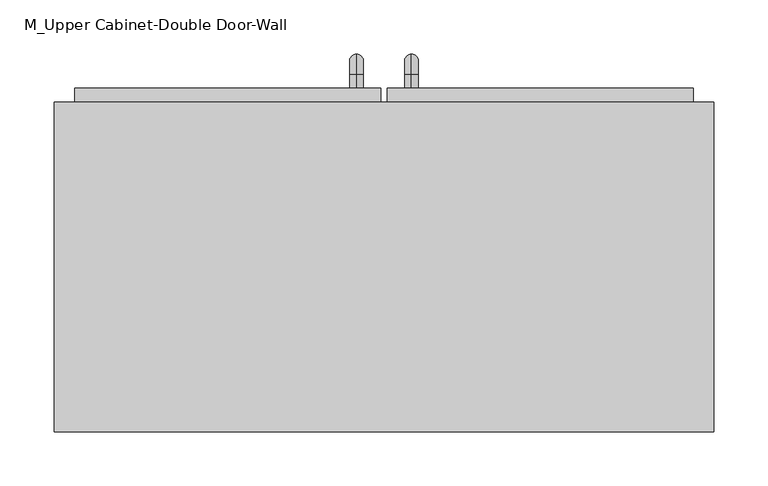
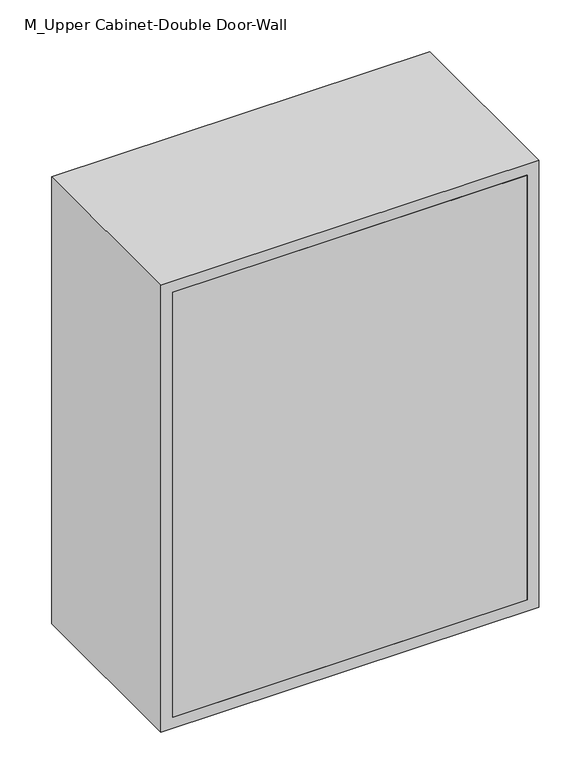
"""IFC4 building model written with IfcOpenShell, lengths in millimetres: furniture geometry, M_Upper Cabinet-Double Door-Wall : 24W X 30H."""

from ifc_helpers import new_model, si_unit, point, frame, origin, place, context, project, spatial, polyline, circle_curve, ellipse_curve, trimmed, outline, extrude, source, transform, mapped, element, save
from ifc_brep_helpers import plane_surface, cylinder_surface, revolved_surface, advanced_brep


def m_upper_cabinet_double_door_wall_c5bb5ff2(model_context):
    return source(origin(), model_context, "Body", "SolidModel", [
        advanced_brep(
        [(55.1711628, 379.4125, 1212.85), (55.1711628, 379.4125, 1225.55), (55.1711628, 392.1125, 1212.85), (55.1711628, 392.1125, 1225.55), (55.1711628, 411.1625, 1206.5), (55.1711628, 398.4625, 1206.5), (55.1711628, 398.4625, 1130.3), (55.1711628, 411.1625, 1130.3), (55.1711628, 392.1125, 1111.25), (55.1711628, 392.1125, 1123.95), (55.1711628, 379.4125, 1123.95), (55.1711628, 379.4125, 1111.25)],
        [
            (0, 1, circle_curve(frame((55.1711628, 379.4125, 1219.2), z_axis=(0.0, -1.0, 0.0), x_axis=(0.0, 0.0, -1.0)), 6.35)),
            (1, 0, circle_curve(frame((55.1711628, 379.4125, 1219.2), z_axis=(0.0, -1.0, 0.0), x_axis=(0.0, 0.0, -1.0)), 6.35)),
            (0, 2),
            (2, 3, circle_curve(frame((55.1711628, 392.1125, 1219.2), z_axis=(0.0, -1.0, 0.0), x_axis=(0.0, 0.0, -1.0)), 6.35)),
            (3, 1),
            (3, 2, circle_curve(frame((55.1711628, 392.1125, 1219.2), z_axis=(0.0, -1.0, 0.0), x_axis=(0.0, 0.0, -1.0)), 6.35)),
            (4, 3, circle_curve(frame((55.1711628, 392.1125, 1206.5), z_axis=(1.0, 0.0, 0.0), x_axis=(0.0, 0.0, 1.0)), 19.05)),
            (2, 5, circle_curve(frame((55.1711628, 392.1125, 1206.5), z_axis=(-1.0, 0.0, 0.0), x_axis=(0.0, 0.0, 1.0)), 6.35)),
            (5, 4, circle_curve(frame((55.1711628, 404.8125, 1206.5), z_axis=(0.0, 0.0, 1.0), x_axis=(0.0, -1.0, 0.0)), 6.35)),
            (4, 5, circle_curve(frame((55.1711628, 404.8125, 1206.5), z_axis=(0.0, 0.0, 1.0), x_axis=(0.0, -1.0, 0.0)), 6.35)),
            (5, 6),
            (6, 7, circle_curve(frame((55.1711628, 404.8125, 1130.3), z_axis=(0.0, 0.0, 1.0), x_axis=(0.0, -1.0, 0.0)), 6.35)),
            (7, 4),
            (7, 6, circle_curve(frame((55.1711628, 404.8125, 1130.3), z_axis=(0.0, 0.0, 1.0), x_axis=(0.0, -1.0, 0.0)), 6.35)),
            (8, 7, circle_curve(frame((55.1711628, 392.1125, 1130.3), z_axis=(1.0, 0.0, 0.0), x_axis=(0.0, 1.0, 0.0)), 19.05)),
            (6, 9, circle_curve(frame((55.1711628, 392.1125, 1130.3), z_axis=(-1.0, 0.0, 0.0), x_axis=(0.0, 1.0, 0.0)), 6.35)),
            (9, 8, circle_curve(frame((55.1711628, 392.1125, 1117.6), z_axis=(0.0, 1.0, 0.0), x_axis=(0.0, 0.0, 1.0)), 6.35)),
            (8, 9, circle_curve(frame((55.1711628, 392.1125, 1117.6), z_axis=(0.0, 1.0, 0.0), x_axis=(0.0, 0.0, 1.0)), 6.35)),
            (10, 11, circle_curve(frame((55.1711628, 379.4125, 1117.6), z_axis=(0.0, -1.0, 0.0), x_axis=(0.0, 0.0, 1.0)), 6.35)),
            (11, 10, circle_curve(frame((55.1711628, 379.4125, 1117.6), z_axis=(0.0, -1.0, 0.0), x_axis=(0.0, 0.0, 1.0)), 6.35)),
            (9, 10),
            (11, 8),
        ],
        [
            plane_surface(frame((48.8211628, 379.4125, 1219.2), z_axis=(0.0, -1.0, 0.0), x_axis=(0.0, 0.0, 1.0))),
            cylinder_surface(frame((55.1711628, 379.4125, 1219.2), z_axis=(0.0, -1.0, 0.0), x_axis=(0.0, 0.0, -1.0)), 6.35),
            revolved_surface(trimmed(ellipse_curve(frame((55.1711628, 392.1125, 1219.2), z_axis=(0.0, -1.0, 0.0), x_axis=(0.0, 0.0, -1.0)), 6.35, 6.35), [point((55.1711628, 392.1125, 1212.85))], [point((55.1711628, 392.1125, 1225.55))], True, "CARTESIAN"), (55.1711628, 392.1125, 1206.5), (-1.0, 0.0, 0.0)),
            revolved_surface(trimmed(ellipse_curve(frame((55.1711628, 392.1125, 1219.2), z_axis=(0.0, -1.0, 0.0), x_axis=(0.0, 0.0, -1.0)), 6.35, 6.35), [point((55.1711628, 392.1125, 1225.55))], [point((55.1711628, 392.1125, 1212.85))], True, "CARTESIAN"), (55.1711628, 392.1125, 1206.5), (-1.0, 0.0, 0.0)),
            cylinder_surface(frame((55.1711628, 404.8125, 1206.5), z_axis=(0.0, 0.0, 1.0), x_axis=(0.0, -1.0, 0.0)), 6.35),
            revolved_surface(trimmed(ellipse_curve(frame((55.1711628, 404.8125, 1130.3), z_axis=(0.0, 0.0, 1.0), x_axis=(0.0, -1.0, 0.0)), 6.35, 6.35), [point((55.1711628, 398.4625, 1130.3))], [point((55.1711628, 411.1625, 1130.3))], True, "CARTESIAN"), (55.1711628, 392.1125, 1130.3), (-1.0, 0.0, 0.0)),
            revolved_surface(trimmed(ellipse_curve(frame((55.1711628, 404.8125, 1130.3), z_axis=(0.0, 0.0, 1.0), x_axis=(0.0, -1.0, 0.0)), 6.35, 6.35), [point((55.1711628, 411.1625, 1130.3))], [point((55.1711628, 398.4625, 1130.3))], True, "CARTESIAN"), (55.1711628, 392.1125, 1130.3), (-1.0, 0.0, 0.0)),
            plane_surface(frame((48.8211628, 379.4125, 1117.6), z_axis=(0.0, -1.0, 0.0), x_axis=(0.0, 0.0, -1.0))),
            cylinder_surface(frame((55.1711628, 392.1125, 1117.6), z_axis=(0.0, 1.0, 0.0), x_axis=(0.0, 0.0, 1.0)), 6.35),
        ],
        [
            (0, [[1, 2]]),
            (1, [[-1, 3, 4, 5]]),
            (1, [[-2, -5, 6, -3]]),
            (2, [[7, -4, 8, 9]]),
            (3, [[-8, -6, -7, 10]]),
            (4, [[-9, 11, 12, 13]]),
            (4, [[-10, -13, 14, -11]]),
            (5, [[15, -12, 16, 17]]),
            (6, [[-16, -14, -15, 18]]),
            (7, [[19, 20]]),
            (8, [[-17, 21, -20, 22]]),
            (8, [[-18, -22, -19, -21]]),
        ],
    ),
        advanced_brep(
        [(4.3711628, 379.4125, 1212.85), (4.3711628, 379.4125, 1225.55), (4.3711628, 392.1125, 1212.85), (4.3711628, 392.1125, 1225.55), (4.3711628, 411.1625, 1206.5), (4.3711628, 398.4625, 1206.5), (4.3711628, 398.4625, 1130.3), (4.3711628, 411.1625, 1130.3), (4.3711628, 392.1125, 1111.25), (4.3711628, 392.1125, 1123.95), (4.3711628, 379.4125, 1123.95), (4.3711628, 379.4125, 1111.25)],
        [
            (0, 1, circle_curve(frame((4.3711628, 379.4125, 1219.2), z_axis=(0.0, -1.0, 0.0), x_axis=(0.0, 0.0, 1.0)), 6.35)),
            (1, 0, circle_curve(frame((4.3711628, 379.4125, 1219.2), z_axis=(0.0, -1.0, 0.0), x_axis=(0.0, 0.0, 1.0)), 6.35)),
            (0, 2),
            (2, 3, circle_curve(frame((4.3711628, 392.1125, 1219.2), z_axis=(0.0, -1.0, 0.0), x_axis=(0.0, 0.0, 1.0)), 6.35)),
            (3, 1),
            (3, 2, circle_curve(frame((4.3711628, 392.1125, 1219.2), z_axis=(0.0, -1.0, 0.0), x_axis=(0.0, 0.0, 1.0)), 6.35)),
            (4, 3, circle_curve(frame((4.3711628, 392.1125, 1206.5), z_axis=(1.0, 0.0, 0.0), x_axis=(0.0, 0.0, 1.0)), 19.05)),
            (2, 5, circle_curve(frame((4.3711628, 392.1125, 1206.5), z_axis=(-1.0, 0.0, 0.0), x_axis=(0.0, 0.0, 1.0)), 6.35)),
            (5, 4, circle_curve(frame((4.3711628, 404.8125, 1206.5), z_axis=(0.0, 0.0, 1.0), x_axis=(0.0, 1.0, 0.0)), 6.35)),
            (4, 5, circle_curve(frame((4.3711628, 404.8125, 1206.5), z_axis=(0.0, 0.0, 1.0), x_axis=(0.0, 1.0, 0.0)), 6.35)),
            (5, 6),
            (6, 7, circle_curve(frame((4.3711628, 404.8125, 1130.3), z_axis=(0.0, 0.0, 1.0), x_axis=(0.0, 1.0, 0.0)), 6.35)),
            (7, 4),
            (7, 6, circle_curve(frame((4.3711628, 404.8125, 1130.3), z_axis=(0.0, 0.0, 1.0), x_axis=(0.0, 1.0, 0.0)), 6.35)),
            (8, 7, circle_curve(frame((4.3711628, 392.1125, 1130.3), z_axis=(1.0, 0.0, 0.0), x_axis=(0.0, 1.0, 0.0)), 19.05)),
            (6, 9, circle_curve(frame((4.3711628, 392.1125, 1130.3), z_axis=(-1.0, 0.0, 0.0), x_axis=(0.0, 1.0, 0.0)), 6.35)),
            (9, 8, circle_curve(frame((4.3711628, 392.1125, 1117.6), z_axis=(0.0, 1.0, 0.0), x_axis=(0.0, 0.0, -1.0)), 6.35)),
            (8, 9, circle_curve(frame((4.3711628, 392.1125, 1117.6), z_axis=(0.0, 1.0, 0.0), x_axis=(0.0, 0.0, -1.0)), 6.35)),
            (10, 11, circle_curve(frame((4.3711628, 379.4125, 1117.6), z_axis=(0.0, -1.0, 0.0), x_axis=(0.0, 0.0, -1.0)), 6.35)),
            (11, 10, circle_curve(frame((4.3711628, 379.4125, 1117.6), z_axis=(0.0, -1.0, 0.0), x_axis=(0.0, 0.0, -1.0)), 6.35)),
            (9, 10),
            (11, 8),
        ],
        [
            plane_surface(frame((-1.9788372, 379.4125, 1219.2), z_axis=(0.0, -1.0, 0.0), x_axis=(0.0, 0.0, 1.0))),
            cylinder_surface(frame((4.3711628, 379.4125, 1219.2), z_axis=(0.0, -1.0, 0.0), x_axis=(0.0, 0.0, 1.0)), 6.35),
            revolved_surface(trimmed(ellipse_curve(frame((4.3711628, 392.1125, 1219.2), z_axis=(0.0, -1.0, 0.0), x_axis=(0.0, 0.0, 1.0)), 6.35, 6.35), [point((4.3711628, 392.1125, 1212.85))], [point((4.3711628, 392.1125, 1225.55))], True, "CARTESIAN"), (4.3711628, 392.1125, 1206.5), (-1.0, 0.0, 0.0)),
            revolved_surface(trimmed(ellipse_curve(frame((4.3711628, 392.1125, 1219.2), z_axis=(0.0, -1.0, 0.0), x_axis=(0.0, 0.0, 1.0)), 6.35, 6.35), [point((4.3711628, 392.1125, 1225.55))], [point((4.3711628, 392.1125, 1212.85))], True, "CARTESIAN"), (4.3711628, 392.1125, 1206.5), (-1.0, 0.0, 0.0)),
            cylinder_surface(frame((4.3711628, 404.8125, 1206.5), z_axis=(0.0, 0.0, 1.0), x_axis=(0.0, 1.0, 0.0)), 6.35),
            revolved_surface(trimmed(ellipse_curve(frame((4.3711628, 404.8125, 1130.3), z_axis=(0.0, 0.0, 1.0), x_axis=(0.0, 1.0, 0.0)), 6.35, 6.35), [point((4.3711628, 398.4625, 1130.3))], [point((4.3711628, 411.1625, 1130.3))], True, "CARTESIAN"), (4.3711628, 392.1125, 1130.3), (-1.0, 0.0, 0.0)),
            revolved_surface(trimmed(ellipse_curve(frame((4.3711628, 404.8125, 1130.3), z_axis=(0.0, 0.0, 1.0), x_axis=(0.0, 1.0, 0.0)), 6.35, 6.35), [point((4.3711628, 411.1625, 1130.3))], [point((4.3711628, 398.4625, 1130.3))], True, "CARTESIAN"), (4.3711628, 392.1125, 1130.3), (-1.0, 0.0, 0.0)),
            plane_surface(frame((-1.9788372, 379.4125, 1117.6), z_axis=(0.0, -1.0, 0.0), x_axis=(0.0, 0.0, -1.0))),
            cylinder_surface(frame((4.3711628, 392.1125, 1117.6), z_axis=(0.0, 1.0, 0.0), x_axis=(0.0, 0.0, -1.0)), 6.35),
        ],
        [
            (0, [[1, 2]]),
            (1, [[-1, 3, 4, 5]]),
            (1, [[-2, -5, 6, -3]]),
            (2, [[7, -4, 8, 9]]),
            (3, [[-8, -6, -7, 10]]),
            (4, [[-9, 11, 12, 13]]),
            (4, [[-10, -13, 14, -11]]),
            (5, [[15, -12, 16, 17]]),
            (6, [[-16, -14, -15, 18]]),
            (7, [[19, 20]]),
            (8, [[-17, 21, -20, 22]]),
            (8, [[-18, -22, -19, -21]]),
        ],
    ),
        extrude(outline(polyline([(32.9461628, 379.4125), (315.5211628, 379.4125), (315.5211628, 347.6625), (32.9461628, 347.6625), (32.9461628, 379.4125)])), frame((0.0, 0.0, 1085.85), z_axis=(0.0, 0.0, 1.0), x_axis=(1.0, 0.0, 0.0)), (0.0, 0.0, 1.0), 723.9),
        extrude(outline(polyline([(-255.9788372, 379.4125), (26.5961628, 379.4125), (26.5961628, 347.6625), (-255.9788372, 347.6625), (-255.9788372, 379.4125)])), frame((0.0, 0.0, 1085.85), z_axis=(0.0, 0.0, 1.0), x_axis=(1.0, 0.0, 0.0)), (0.0, 0.0, 1.0), 723.9),
        extrude(outline(polyline([(315.5211628, 61.9125), (-255.9788372, 61.9125), (-255.9788372, 80.9625), (315.5211628, 80.9625), (315.5211628, 61.9125)])), frame((0.0, 0.0, 1085.85), z_axis=(0.0, 0.0, 1.0), x_axis=(1.0, 0.0, 0.0)), (0.0, 0.0, 1.0), 723.9),
        extrude(outline(polyline([(1828.8, -275.0288372), (1066.8, -275.0288372), (1066.8, 334.5711628), (1828.8, 334.5711628), (1828.8, -275.0288372)]), holes=[polyline([(1809.75, -255.9788372), (1809.75, 315.5211628), (1085.85, 315.5211628), (1085.85, -255.9788372), (1809.75, -255.9788372)])]), frame((0.0, 61.9125, 0.0), z_axis=(0.0, 1.0, 0.0), x_axis=(0.0, 0.0, 1.0)), (0.0, 0.0, 1.0), 304.8),
    ])


if __name__ == "__main__":
    model = new_model("IFC4")
    model_context = context("Model", 3, world=origin())
    ifc_project = project(units=[si_unit("LENGTHUNIT", "METRE", prefix="MILLI")], contexts=[model_context])
    site = spatial("IfcSite", under=ifc_project)
    building = spatial("IfcBuilding", under=site)
    placement = place(None, origin())
    m_upper_cabinet_double_door_wall_shape = m_upper_cabinet_double_door_wall_c5bb5ff2(model_context)
    element("IfcFurniture", 1, ObjectType="M_Upper Cabinet-Double Door-Wall : 24W X 30H", at=placement, inside=building, context=model_context, shape_type="MappedRepresentation", body=[
        mapped(m_upper_cabinet_double_door_wall_shape, transform((0.0, 0.0, 0.0), x_axis=(1.0, 0.0, 0.0), y_axis=(0.0, 1.0, 0.0), z_axis=(0.0, 0.0, 1.0))),
    ])
    save(model, "model.ifc")

# Revit data of these elements
# Type "M_Upper Cabinet-Double Door-Wall : 24W X 30H"
#   Depth = 1' - 0"
#   Height = 2' - 6"
#   Top Of Cabinet = 6' - 0"
#   Width = 2' - 0"
#   Cabinet Material = none
#   Door/Drawer Material = none
#   Handle Material = Cabinets - Handles
# Element 1 (IfcFurniture, "M_Upper Cabinet-Double Door-Wall : 24W X 30H")
#   Materials on its faces: "Cabinets", "Cabinets - Handles"
# Materials
#   "Cabinets - Handles": class "Metal", colour RGB 57 57 57, transparency 0
#   "Cabinets": class "Miscellaneous", colour RGB 249 249 249, transparency 0
